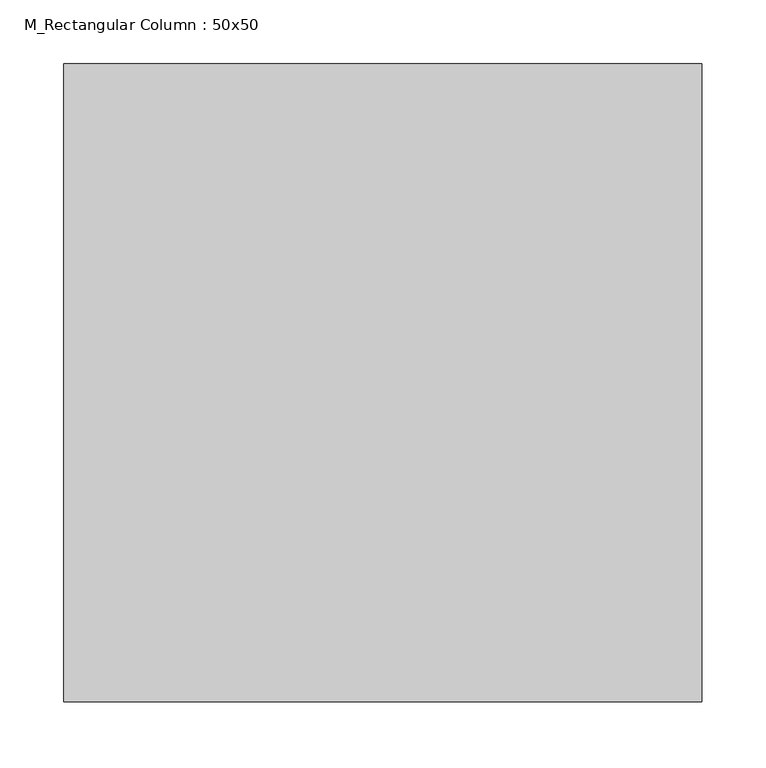
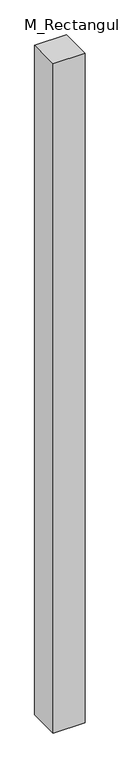
"""IFC4 building model written with IfcOpenShell, lengths in millimetres: column geometry, M_Rectangular Column : 50x50."""

from ifc_helpers import new_model, si_unit, frame, origin, place, context, project, spatial, polyline, outline, extrude, source, transform, mapped, element, save


def m_rectangular_column_50x50_3a95f3c9(model_context):
    return source(origin(), model_context, "Body", "SweptSolid", [
        extrude(outline(polyline([(250.0, 250.0), (250.0, -250.0), (-250.0, -250.0), (-250.0, 250.0), (250.0, 250.0)])), frame((0.0, 0.0, -3200.0), z_axis=(0.0, 0.0, 1.0), x_axis=(1.0, 0.0, 0.0)), (0.0, 0.0, 1.0), 11100.0),
    ])


if __name__ == "__main__":
    model = new_model("IFC4")
    model_context = context("Model", 3, world=origin())
    ifc_project = project(units=[si_unit("LENGTHUNIT", "METRE", prefix="MILLI")], contexts=[model_context])
    site = spatial("IfcSite", under=ifc_project)
    building = spatial("IfcBuilding", under=site)
    placement = place(None, origin())
    m_rectangular_column_50x50_shape = m_rectangular_column_50x50_3a95f3c9(model_context)
    element("IfcColumn", 1, ObjectType="M_Rectangular Column : 50x50", at=placement, inside=building, context=model_context, shape_type="MappedRepresentation", body=[
        mapped(m_rectangular_column_50x50_shape, transform((0.0, 0.0, 0.0), x_axis=(1.0, 0.0, 0.0), y_axis=(0.0, 1.0, 0.0), z_axis=(0.0, 0.0, 1.0))),
    ])
    save(model, "model.ifc")

# Revit data of these elements
# Type "M_Rectangular Column : 50x50"
#   Depth = 50 cm
#   Offset Base = 0 cm
#   Offset Top = 0 cm
#   Width = 50 cm
#   Material = none
